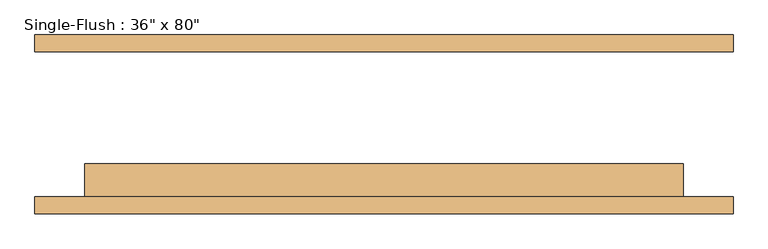
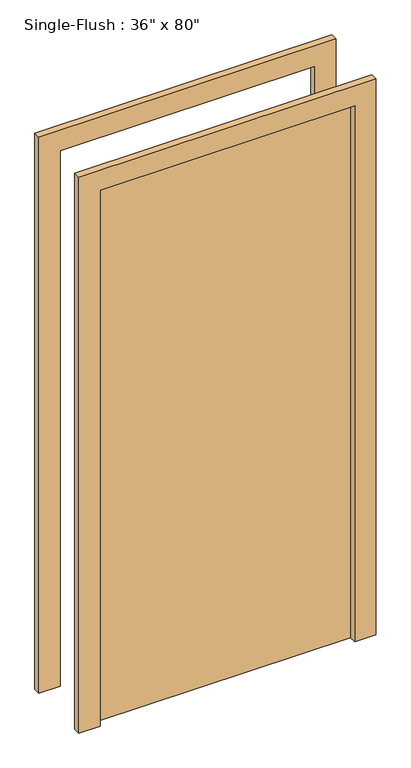
"""IFC4 building model written with IfcOpenShell, lengths in millimetres: door geometry."""

from ifc_helpers import new_model, si_unit, frame, origin, origin_with_axes, place, context, project, spatial, polyline, outline, extrude, source, transform, mapped, element, save


def door_d5b76e51(model_context):
    return source(origin(), model_context, "Body", "SweptSolid", [
        extrude(outline(polyline([(2108.2, -533.4), (0.0, -533.4), (0.0, -457.2), (2032.0, -457.2), (2032.0, 457.2), (0.0, 457.2), (0.0, 533.4), (2108.2, 533.4), (2108.2, -533.4)])), frame((0.0, -136.525, 0.0), z_axis=(0.0, 1.0, 0.0), x_axis=(0.0, 0.0, 1.0)), (0.0, 0.0, 1.0), 25.4),
        extrude(outline(polyline([(2108.2, 533.4), (2108.2, -533.4), (0.0, -533.4), (0.0, -457.2), (2032.0, -457.2), (2032.0, 457.2), (0.0, 457.2), (0.0, 533.4), (2108.2, 533.4)])), frame((0.0, 111.125, 0.0), z_axis=(0.0, 1.0, 0.0), x_axis=(0.0, 0.0, 1.0)), (0.0, 0.0, 1.0), 25.4),
        extrude(outline(polyline([(457.2, -60.325), (457.2, -111.125), (-457.2, -111.125), (-457.2, -60.325), (457.2, -60.325)])), origin_with_axes(), (0.0, 0.0, 1.0), 2032.0),
    ])


if __name__ == "__main__":
    model = new_model("IFC4")
    model_context = context("Model", 3, world=origin())
    ifc_project = project(units=[si_unit("LENGTHUNIT", "METRE", prefix="MILLI")], contexts=[model_context])
    site = spatial("IfcSite", under=ifc_project)
    building = spatial("IfcBuilding", under=site)
    placement = place(None, origin())
    door_shape = door_d5b76e51(model_context)
    element("IfcDoor", 1, ObjectType="Single-Flush : 36\" x 80\"", at=placement, inside=building, context=model_context, shape_type="MappedRepresentation", body=[
        mapped(door_shape, transform((0.0, 0.0, 0.0), x_axis=(1.0, 0.0, 0.0), y_axis=(0.0, 1.0, 0.0), z_axis=(0.0, 0.0, 1.0))),
    ])
    save(model, "model.ifc")

# Revit data of these elements
# Type "Single-Flush : 36\" x 80\""
#   Type Mark = "13"
#   Construction Type Id = "MDOOR"
#   Assembly Code = "C1020"
#   Analytic Construction = "Metal"
#   Thickness = 0' - 2"
#   Heat Transfer Coefficient (U) = 3.7021 W/(m²·K)
#   Height = 6' - 8"
#   Trim Projection Ext = 0' - 1"
#   Trim Projection Int = 0' - 1"
#   Trim Width = 0' - 3"
#   Width = 3' - 0"
#   Door Material = INTERIOR GRADE ALUMINUM STOREFRONT W/ SAFETY GLAZING
#   Frame Material = INTERIOR GRADE ALUMINUM STOREFRONT W/ SAFETY GLAZING
#   Visual Light Transmittance = 0
#   Solar Heat Gain Coefficient = 0
#   Function = (empty or 0)
#   Wall Closure = (empty or 0)
# Element 1 (IfcDoor, "Single-Flush : 36\" x 80\"")
#   Materials on its faces: "INTERIOR GRADE ALUMINUM STOREFRONT W/ SAFETY GLAZING"
# Materials
#   "INTERIOR GRADE ALUMINUM STOREFRONT W/ SAFETY GLAZING": class "Metal", colour RGB 226 226 226, transparency 0, Description = "Aluminum 6061", Cost = 0
